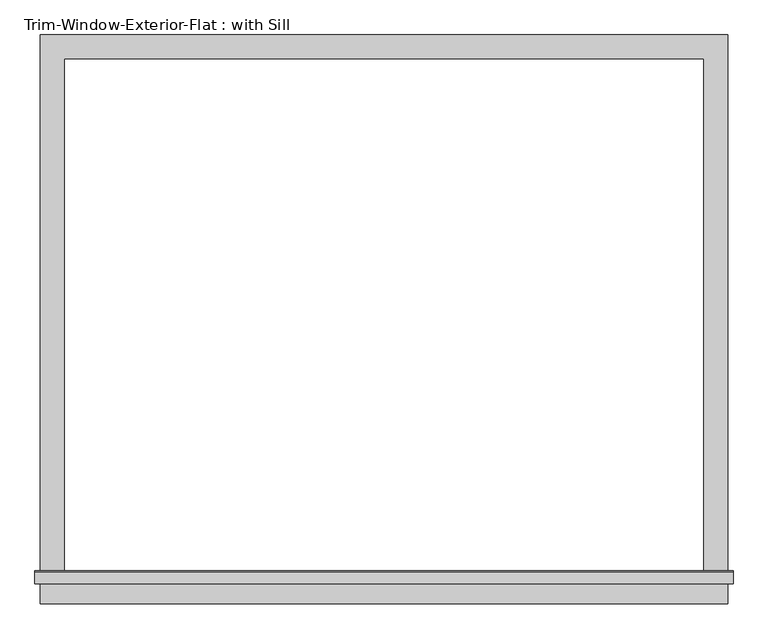
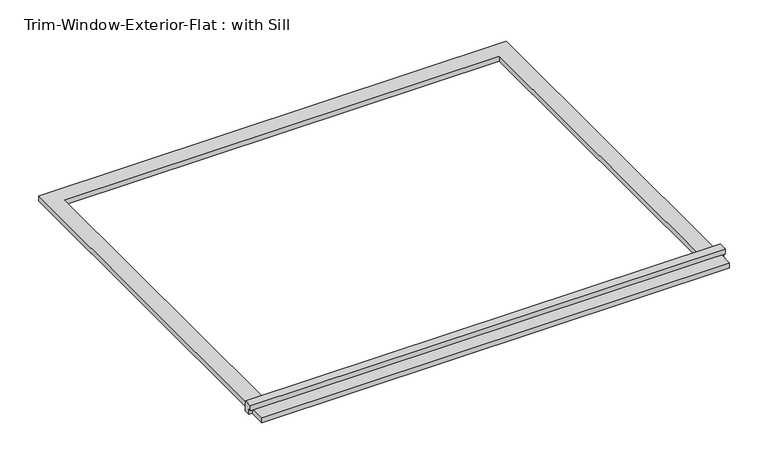
"""IFC4 building model written with IfcOpenShell, lengths in millimetres: proxy geometry, Trim-Window-Exterior-Flat : with Sill."""

import ifcopenshell
import ifcopenshell.guid

model = None  # the IFC model being written
_history = None  # IfcOwnerHistory: only IFC2X3 demands one
_inside = {}  # id of a spatial element -> (the spatial element, [elements in it])
_under = {}  # id of a project, library or spatial element -> (it, [spatial elements below it])
_declared = {}  # id of a project -> (the project, [libraries it declares])
_typed = {}  # id of a type object -> (the type object, [elements of that type])
_made_of = {}  # id of a material, layer set ... -> (it, [elements and type objects made of it])


def new_model(schema):
    """Start an empty IFC model of exactly this schema.

    Asked for "IFC4X3", IfcOpenShell would pick the latest addendum, in which some entities
    have other attributes; the version numbers below select the first issue.
    IFC2X3 requires an IfcOwnerHistory on every rooted entity: one is made here for all.
    """
    global model, _history
    if schema == "IFC4X3":
        model = ifcopenshell.file(schema_version=(4, 3, 0, 0))
    else:
        model = ifcopenshell.file(schema=schema)
    _inside.clear()
    _under.clear()
    _declared.clear()
    _typed.clear()
    _made_of.clear()
    _history = None
    if model.schema == "IFC2X3":
        org = make("IfcOrganization", Name="unknown")
        user = make(
            "IfcPersonAndOrganization",
            ThePerson=make("IfcPerson", FamilyName="unknown"),
            TheOrganization=org,
        )
        app = make(
            "IfcApplication",
            ApplicationDeveloper=org,
            Version="unknown",
            ApplicationFullName="unknown",
            ApplicationIdentifier="unknown",
        )
        _history = make(
            "IfcOwnerHistory",
            OwningUser=user,
            OwningApplication=app,
            ChangeAction="ADDED",
            CreationDate=0,
        )
    return model


def make(cls, **values):
    """One entity of the class cls with the attributes given. An attribute that is None is left unset."""
    return model.create_entity(
        cls, **{name: value for name, value in values.items() if value is not None}
    )


def rooted(cls, **values):
    """An entity with a GlobalId (a new one), such as an element, a storey or a relation."""
    return make(cls, GlobalId=ifcopenshell.guid.new(), OwnerHistory=_history, **values)


def si_unit(unit_type, name, prefix=None):
    """IfcSIUnit, for example si_unit("LENGTHUNIT", "METRE", prefix="MILLI")."""
    return make("IfcSIUnit", UnitType=unit_type, Prefix=prefix, Name=name)


def assignment(units):
    """IfcUnitAssignment: the units of a project."""
    return None if units is None else make("IfcUnitAssignment", Units=units)


def point(xyz):
    """IfcCartesianPoint."""
    return None if xyz is None else make("IfcCartesianPoint", Coordinates=xyz)


def direction(xyz):
    """IfcDirection."""
    return None if xyz is None else make("IfcDirection", DirectionRatios=xyz)


def frame(location, z_axis=None, x_axis=None):
    """IfcAxis2Placement3D, a coordinate frame: its origin and axes. An axis left out is left unset."""
    return make(
        "IfcAxis2Placement3D",
        Location=point(location),
        Axis=direction(z_axis),
        RefDirection=direction(x_axis),
    )


def origin():
    """The frame at (0, 0, 0) with its axes left unset."""
    return frame((0.0, 0.0, 0.0))


def origin_with_axes():
    """The frame at (0, 0, 0) with the z axis (0, 0, 1) and the x axis (1, 0, 0) written out."""
    return frame((0.0, 0.0, 0.0), z_axis=(0.0, 0.0, 1.0), x_axis=(1.0, 0.0, 0.0))


def place(relative_to, where):
    """IfcLocalPlacement: puts the frame where relative to a parent placement (None: the world)."""
    return make(
        "IfcLocalPlacement", PlacementRelTo=relative_to, RelativePlacement=where
    )


def context(
    kind, dimensions, precision=None, world=None, true_north=None, identifier=None
):
    """IfcGeometricRepresentationContext, for example the 3D "Model" context."""
    return make(
        "IfcGeometricRepresentationContext",
        ContextIdentifier=identifier,
        ContextType=kind,
        CoordinateSpaceDimension=dimensions,
        Precision=precision,
        WorldCoordinateSystem=world,
        TrueNorth=true_north,
    )


def project(units=None, contexts=None):
    """IfcProject with its units and contexts."""
    return rooted(
        "IfcProject",
        Name="project",
        RepresentationContexts=contexts,
        UnitsInContext=assignment(units),
    )


def spatial(cls, under=None, at=None, **own):
    """A site, building, storey or space (cls), placed at a placement, below another one or the project."""
    s = rooted(cls, ObjectPlacement=at, **own)
    if under is not None:
        _under.setdefault(under.id(), (under, []))[1].append(s)
    return s


def polyline(points):
    """IfcPolyline through the points."""
    return make("IfcPolyline", Points=[point(p) for p in points])


def outline(outer, holes=None, kind="AREA"):
    """IfcArbitraryClosedProfileDef: a profile drawn as a closed curve; with holes, ...WithVoids."""
    if holes is None:
        return make("IfcArbitraryClosedProfileDef", ProfileType=kind, OuterCurve=outer)
    return make(
        "IfcArbitraryProfileDefWithVoids",
        ProfileType=kind,
        OuterCurve=outer,
        InnerCurves=holes,
    )


def extrude(swept, where, along, depth):
    """IfcExtrudedAreaSolid: the profile swept, set in the frame where, extruded along a direction by depth."""
    return make(
        "IfcExtrudedAreaSolid",
        SweptArea=swept,
        Position=where,
        ExtrudedDirection=direction(along),
        Depth=depth,
    )


def shape(context_of_items, identifier, shape_type, items):
    """IfcShapeRepresentation: the items that make up one representation, for example the "Body"."""
    return make(
        "IfcShapeRepresentation",
        ContextOfItems=context_of_items,
        RepresentationIdentifier=identifier,
        RepresentationType=shape_type,
        Items=items,
    )


def source(mapping_origin, context_of_items, identifier, shape_type, items):
    """IfcRepresentationMap: a shape defined once, which mapped items show again and again."""
    return make(
        "IfcRepresentationMap",
        MappingOrigin=mapping_origin,
        MappedRepresentation=shape(context_of_items, identifier, shape_type, items),
    )


def transform(
    local_origin,
    x_axis=None,
    y_axis=None,
    z_axis=None,
    scale=None,
    scale2=None,
    scale3=None,
    uniform=True,
):
    """IfcCartesianTransformationOperator3D, or its non-uniform kind. x_axis, y_axis, z_axis: its Axis1, 2, 3."""
    if uniform:
        return make(
            "IfcCartesianTransformationOperator3D",
            Axis1=direction(x_axis),
            Axis2=direction(y_axis),
            LocalOrigin=point(local_origin),
            Scale=scale,
            Axis3=direction(z_axis),
        )
    return make(
        "IfcCartesianTransformationOperator3DnonUniform",
        Axis1=direction(x_axis),
        Axis2=direction(y_axis),
        LocalOrigin=point(local_origin),
        Scale=scale,
        Axis3=direction(z_axis),
        Scale2=scale2,
        Scale3=scale3,
    )


def mapped(mapping_source, mapping_target):
    """IfcMappedItem: shows the shape of a source again, moved by a transform."""
    return make(
        "IfcMappedItem", MappingSource=mapping_source, MappingTarget=mapping_target
    )


def made_of(thing, what):
    """Note that an element or type object is made of a material, layer set ...; save() writes the relation."""
    if what is not None:
        _made_of.setdefault(what.id(), (what, []))[1].append(thing)
    return thing


def element(
    cls,
    number,
    at=None,
    inside=None,
    cuts=None,
    type_object=None,
    material=None,
    context=None,
    identifier="Body",
    shape_type=None,
    held_by="IfcProductDefinitionShape",
    body=None,
    shapes=None,
    **own,
):
    """One element of the class cls, such as IfcWall. Its Tag is "e" and its number.

    at: its placement. inside: the storey or other place that contains it. cuts: it is an
    opening in that element (IfcRelVoidsElement). A single representation is given by context,
    identifier, shape_type and body (its items); several are given by shapes. held_by: the class
    of the entity that holds the representations. save() writes the other relations.
    """
    e = rooted(cls, Tag="e%d" % number, ObjectPlacement=at, **own)
    if body is not None:
        shapes = [shape(context, identifier, shape_type, body)]
    if shapes is not None:
        e.Representation = make(held_by, Representations=shapes)
    if inside is not None:
        _inside.setdefault(inside.id(), (inside, []))[1].append(e)
    if cuts is not None:
        rooted(
            "IfcRelVoidsElement", RelatingBuildingElement=cuts, RelatedOpeningElement=e
        )
    if type_object is not None:
        _typed.setdefault(type_object.id(), (type_object, []))[1].append(e)
    return made_of(e, material)


def aggregate(whole, parts):
    """IfcRelAggregates: a whole, such as a stair, and the parts it consists of."""
    return rooted("IfcRelAggregates", RelatingObject=whole, RelatedObjects=parts)


def save(model, path):
    """Write the relations noted so far, then the file.

    IfcRelAggregates (storeys below a building ...), IfcRelContainedInSpatialStructure (elements
    in a storey), IfcRelDefinesByType, IfcRelAssociatesMaterial and IfcRelDeclares: one each for
    every whole, place, type object, material and project.
    """
    for whole, parts in _under.values():
        aggregate(whole, parts)
    for where, things in _inside.values():
        rooted(
            "IfcRelContainedInSpatialStructure",
            RelatedElements=things,
            RelatingStructure=where,
        )
    for kind, things in _typed.values():
        rooted("IfcRelDefinesByType", RelatedObjects=things, RelatingType=kind)
    for what, things in _made_of.values():
        rooted("IfcRelAssociatesMaterial", RelatedObjects=things, RelatingMaterial=what)
    for by, libraries in _declared.values():
        rooted("IfcRelDeclares", RelatingContext=by, RelatedDefinitions=libraries)
    model.write(path)


def trim_window_exterior_flat_with_sill_7631c5ba(model_context):
    return source(origin(), model_context, "Body", "SweptSolid", [
        extrude(outline(polyline([(819.15, -1241.3823709), (819.15, -1298.5323709), (-819.15, -1298.5323709), (-819.15, -1241.3823709), (819.15, -1241.3823709)])), origin_with_axes(), (0.0, 0.0, 1.0), 19.05),
        extrude(outline(polyline([(-1250.95, 38.1), (-1221.6580645, 38.1), (-1219.2, 19.05), (-1219.2, 0.0), (-1241.3823709, 0.0), (-1241.3823709, 19.05), (-1250.95, 19.05), (-1250.95, 38.1)])), frame((-831.85, 0.0, 0.0), z_axis=(1.0, 0.0, 0.0), x_axis=(0.0, 1.0, 0.0)), (0.0, 0.0, 1.0), 1663.7),
        extrude(outline(polyline([(-819.15, 57.15), (819.15, 57.15), (819.15, -1219.2), (762.0, -1219.2), (762.0, 0.0), (-762.0, 0.0), (-762.0, -1219.2), (-819.15, -1219.2), (-819.15, 57.15)])), origin_with_axes(), (0.0, 0.0, 1.0), 19.05),
    ])


if __name__ == "__main__":
    model = new_model("IFC4")
    model_context = context("Model", 3, world=origin())
    ifc_project = project(units=[si_unit("LENGTHUNIT", "METRE", prefix="MILLI")], contexts=[model_context])
    site = spatial("IfcSite", under=ifc_project)
    building = spatial("IfcBuilding", under=site)
    placement = place(None, origin())
    trim_window_exterior_flat_with_sill_shape = trim_window_exterior_flat_with_sill_7631c5ba(model_context)
    element("IfcBuildingElementProxy", 1, Name="Trim-Window-Exterior-Flat : with Sill", ObjectType="Trim-Window-Exterior-Flat : with Sill", at=placement, inside=building, context=model_context, shape_type="MappedRepresentation", body=[
        mapped(trim_window_exterior_flat_with_sill_shape, transform((0.0, 0.0, 0.0), x_axis=(1.0, 0.0, 0.0), y_axis=(0.0, 1.0, 0.0), z_axis=(0.0, 0.0, 1.0))),
    ])
    save(model, "model.ifc")

# Revit data of these elements
# Project information
#   Project Issue Date = "Issue Date"
#   Project Status = "Project Status"
#   Client Name = "Owner"
#   Project Address = "Enter address here"
#   Project Name = "Project Name"
#   Project Number = "Project Number"
# Type "Trim-Window-Exterior-Flat : with Sill"
#   Trim Width = 0' - 2 1/4"
#   Trim Thickness_Picture Frame = 0' - 1 1/4"
#   Trim Thickness_with Sill = 0' - 0 3/4"
#   Sill Thickness = 0' - 1 1/4"
#   Opening Width [instance default] = 2' - 0"
#   Opening Height [instance default] = 3' - 0"
#   Default Elevation = 4' - 0"
#   Sill = yes
#   Picture Frame = no
#   Trim Material [instance default] = none
# Element 1 (IfcBuildingElementProxy, "Trim-Window-Exterior-Flat : with Sill")
#   Opening Width = 5' - 0"
#   Opening Height = 4' - 0"
#   Trim Material = Clad - White
#   Materials on its faces: "Clad - White"
# Materials
#   "Clad - White": class "Wood", colour RGB 242 242 238, transparency 0, Cost = 0
